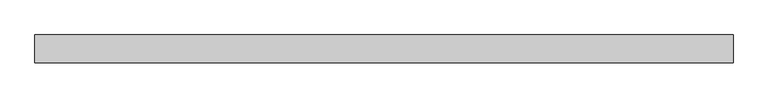
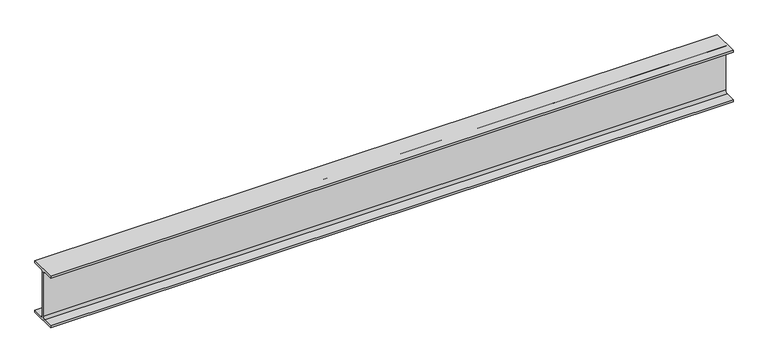
"""IFC4 building model written with IfcOpenShell, lengths in millimetres: beam geometry, 0912_Steel Framing_H-KSD3502 : H_SB_ASB_H-250x125x6x9."""

import ifcopenshell
import ifcopenshell.guid

model = None  # the IFC model being written
_history = None  # IfcOwnerHistory: only IFC2X3 demands one
_inside = {}  # id of a spatial element -> (the spatial element, [elements in it])
_under = {}  # id of a project, library or spatial element -> (it, [spatial elements below it])
_declared = {}  # id of a project -> (the project, [libraries it declares])
_typed = {}  # id of a type object -> (the type object, [elements of that type])
_made_of = {}  # id of a material, layer set ... -> (it, [elements and type objects made of it])


def new_model(schema):
    """Start an empty IFC model of exactly this schema.

    Asked for "IFC4X3", IfcOpenShell would pick the latest addendum, in which some entities
    have other attributes; the version numbers below select the first issue.
    IFC2X3 requires an IfcOwnerHistory on every rooted entity: one is made here for all.
    """
    global model, _history
    if schema == "IFC4X3":
        model = ifcopenshell.file(schema_version=(4, 3, 0, 0))
    else:
        model = ifcopenshell.file(schema=schema)
    _inside.clear()
    _under.clear()
    _declared.clear()
    _typed.clear()
    _made_of.clear()
    _history = None
    if model.schema == "IFC2X3":
        org = make("IfcOrganization", Name="unknown")
        user = make(
            "IfcPersonAndOrganization",
            ThePerson=make("IfcPerson", FamilyName="unknown"),
            TheOrganization=org,
        )
        app = make(
            "IfcApplication",
            ApplicationDeveloper=org,
            Version="unknown",
            ApplicationFullName="unknown",
            ApplicationIdentifier="unknown",
        )
        _history = make(
            "IfcOwnerHistory",
            OwningUser=user,
            OwningApplication=app,
            ChangeAction="ADDED",
            CreationDate=0,
        )
    return model


def make(cls, **values):
    """One entity of the class cls with the attributes given. An attribute that is None is left unset."""
    return model.create_entity(
        cls, **{name: value for name, value in values.items() if value is not None}
    )


def rooted(cls, **values):
    """An entity with a GlobalId (a new one), such as an element, a storey or a relation."""
    return make(cls, GlobalId=ifcopenshell.guid.new(), OwnerHistory=_history, **values)


def si_unit(unit_type, name, prefix=None):
    """IfcSIUnit, for example si_unit("LENGTHUNIT", "METRE", prefix="MILLI")."""
    return make("IfcSIUnit", UnitType=unit_type, Prefix=prefix, Name=name)


def assignment(units):
    """IfcUnitAssignment: the units of a project."""
    return None if units is None else make("IfcUnitAssignment", Units=units)


def point(xyz):
    """IfcCartesianPoint."""
    return None if xyz is None else make("IfcCartesianPoint", Coordinates=xyz)


def direction(xyz):
    """IfcDirection."""
    return None if xyz is None else make("IfcDirection", DirectionRatios=xyz)


def frame(location, z_axis=None, x_axis=None):
    """IfcAxis2Placement3D, a coordinate frame: its origin and axes. An axis left out is left unset."""
    return make(
        "IfcAxis2Placement3D",
        Location=point(location),
        Axis=direction(z_axis),
        RefDirection=direction(x_axis),
    )


def frame_2d(location, x_axis=None):
    """IfcAxis2Placement2D, a coordinate frame in the plane: its origin and x axis."""
    return make(
        "IfcAxis2Placement2D", Location=point(location), RefDirection=direction(x_axis)
    )


def origin():
    """The frame at (0, 0, 0) with its axes left unset."""
    return frame((0.0, 0.0, 0.0))


def place(relative_to, where):
    """IfcLocalPlacement: puts the frame where relative to a parent placement (None: the world)."""
    return make(
        "IfcLocalPlacement", PlacementRelTo=relative_to, RelativePlacement=where
    )


def context(
    kind, dimensions, precision=None, world=None, true_north=None, identifier=None
):
    """IfcGeometricRepresentationContext, for example the 3D "Model" context."""
    return make(
        "IfcGeometricRepresentationContext",
        ContextIdentifier=identifier,
        ContextType=kind,
        CoordinateSpaceDimension=dimensions,
        Precision=precision,
        WorldCoordinateSystem=world,
        TrueNorth=true_north,
    )


def project(units=None, contexts=None):
    """IfcProject with its units and contexts."""
    return rooted(
        "IfcProject",
        Name="project",
        RepresentationContexts=contexts,
        UnitsInContext=assignment(units),
    )


def spatial(cls, under=None, at=None, **own):
    """A site, building, storey or space (cls), placed at a placement, below another one or the project."""
    s = rooted(cls, ObjectPlacement=at, **own)
    if under is not None:
        _under.setdefault(under.id(), (under, []))[1].append(s)
    return s


def polyline(points):
    """IfcPolyline through the points."""
    return make("IfcPolyline", Points=[point(p) for p in points])


def circle_curve(where, radius):
    """IfcCircle in the frame where."""
    return make("IfcCircle", Position=where, Radius=radius)


def trimmed(basis, trim1, trim2, sense, master):
    """IfcTrimmedCurve: the piece of a basis curve between two trims."""
    return make(
        "IfcTrimmedCurve",
        BasisCurve=basis,
        Trim1=trim1,
        Trim2=trim2,
        SenseAgreement=sense,
        MasterRepresentation=master,
    )


def segment(curve, same_sense, transition):
    """IfcCompositeCurveSegment."""
    return make(
        "IfcCompositeCurveSegment",
        Transition=transition,
        SameSense=same_sense,
        ParentCurve=curve,
    )


def composite_curve(segments, self_intersect=None):
    """IfcCompositeCurve: segments joined end to end."""
    return make("IfcCompositeCurve", Segments=segments, SelfIntersect=self_intersect)


def outline(outer, holes=None, kind="AREA"):
    """IfcArbitraryClosedProfileDef: a profile drawn as a closed curve; with holes, ...WithVoids."""
    if holes is None:
        return make("IfcArbitraryClosedProfileDef", ProfileType=kind, OuterCurve=outer)
    return make(
        "IfcArbitraryProfileDefWithVoids",
        ProfileType=kind,
        OuterCurve=outer,
        InnerCurves=holes,
    )


def extrude(swept, where, along, depth):
    """IfcExtrudedAreaSolid: the profile swept, set in the frame where, extruded along a direction by depth."""
    return make(
        "IfcExtrudedAreaSolid",
        SweptArea=swept,
        Position=where,
        ExtrudedDirection=direction(along),
        Depth=depth,
    )


def shape(context_of_items, identifier, shape_type, items):
    """IfcShapeRepresentation: the items that make up one representation, for example the "Body"."""
    return make(
        "IfcShapeRepresentation",
        ContextOfItems=context_of_items,
        RepresentationIdentifier=identifier,
        RepresentationType=shape_type,
        Items=items,
    )


def source(mapping_origin, context_of_items, identifier, shape_type, items):
    """IfcRepresentationMap: a shape defined once, which mapped items show again and again."""
    return make(
        "IfcRepresentationMap",
        MappingOrigin=mapping_origin,
        MappedRepresentation=shape(context_of_items, identifier, shape_type, items),
    )


def transform(
    local_origin,
    x_axis=None,
    y_axis=None,
    z_axis=None,
    scale=None,
    scale2=None,
    scale3=None,
    uniform=True,
):
    """IfcCartesianTransformationOperator3D, or its non-uniform kind. x_axis, y_axis, z_axis: its Axis1, 2, 3."""
    if uniform:
        return make(
            "IfcCartesianTransformationOperator3D",
            Axis1=direction(x_axis),
            Axis2=direction(y_axis),
            LocalOrigin=point(local_origin),
            Scale=scale,
            Axis3=direction(z_axis),
        )
    return make(
        "IfcCartesianTransformationOperator3DnonUniform",
        Axis1=direction(x_axis),
        Axis2=direction(y_axis),
        LocalOrigin=point(local_origin),
        Scale=scale,
        Axis3=direction(z_axis),
        Scale2=scale2,
        Scale3=scale3,
    )


def mapped(mapping_source, mapping_target):
    """IfcMappedItem: shows the shape of a source again, moved by a transform."""
    return make(
        "IfcMappedItem", MappingSource=mapping_source, MappingTarget=mapping_target
    )


def made_of(thing, what):
    """Note that an element or type object is made of a material, layer set ...; save() writes the relation."""
    if what is not None:
        _made_of.setdefault(what.id(), (what, []))[1].append(thing)
    return thing


def element(
    cls,
    number,
    at=None,
    inside=None,
    cuts=None,
    type_object=None,
    material=None,
    context=None,
    identifier="Body",
    shape_type=None,
    held_by="IfcProductDefinitionShape",
    body=None,
    shapes=None,
    **own,
):
    """One element of the class cls, such as IfcWall. Its Tag is "e" and its number.

    at: its placement. inside: the storey or other place that contains it. cuts: it is an
    opening in that element (IfcRelVoidsElement). A single representation is given by context,
    identifier, shape_type and body (its items); several are given by shapes. held_by: the class
    of the entity that holds the representations. save() writes the other relations.
    """
    e = rooted(cls, Tag="e%d" % number, ObjectPlacement=at, **own)
    if body is not None:
        shapes = [shape(context, identifier, shape_type, body)]
    if shapes is not None:
        e.Representation = make(held_by, Representations=shapes)
    if inside is not None:
        _inside.setdefault(inside.id(), (inside, []))[1].append(e)
    if cuts is not None:
        rooted(
            "IfcRelVoidsElement", RelatingBuildingElement=cuts, RelatedOpeningElement=e
        )
    if type_object is not None:
        _typed.setdefault(type_object.id(), (type_object, []))[1].append(e)
    return made_of(e, material)


def aggregate(whole, parts):
    """IfcRelAggregates: a whole, such as a stair, and the parts it consists of."""
    return rooted("IfcRelAggregates", RelatingObject=whole, RelatedObjects=parts)


def save(model, path):
    """Write the relations noted so far, then the file.

    IfcRelAggregates (storeys below a building ...), IfcRelContainedInSpatialStructure (elements
    in a storey), IfcRelDefinesByType, IfcRelAssociatesMaterial and IfcRelDeclares: one each for
    every whole, place, type object, material and project.
    """
    for whole, parts in _under.values():
        aggregate(whole, parts)
    for where, things in _inside.values():
        rooted(
            "IfcRelContainedInSpatialStructure",
            RelatedElements=things,
            RelatingStructure=where,
        )
    for kind, things in _typed.values():
        rooted("IfcRelDefinesByType", RelatedObjects=things, RelatingType=kind)
    for what, things in _made_of.values():
        rooted("IfcRelAssociatesMaterial", RelatedObjects=things, RelatingMaterial=what)
    for by, libraries in _declared.values():
        rooted("IfcRelDeclares", RelatingContext=by, RelatedDefinitions=libraries)
    model.write(path)


def beam_d1df00b5(model_context):
    return source(origin(), model_context, "Body", "SweptSolid", [
        extrude(outline(composite_curve([segment(polyline([(62.5, -116.0), (62.5, -125.0), (-62.5, -125.0), (-62.5, -116.0), (-15.0, -116.0)]), True, "CONTINUOUS"), segment(trimmed(circle_curve(frame_2d((-15.0, -104.0)), 12.0), [point((-15.0, -116.0))], [point((-3.0, -104.0))], True, "CARTESIAN"), True, "CONTINUOUS"), segment(polyline([(-3.0, -104.0), (-3.0, 104.0)]), True, "CONTINUOUS"), segment(trimmed(circle_curve(frame_2d((-15.0, 104.0)), 12.0), [point((-3.0, 104.0))], [point((-15.0, 116.0))], True, "CARTESIAN"), True, "CONTINUOUS"), segment(polyline([(-15.0, 116.0), (-62.5, 116.0), (-62.5, 125.0), (62.5, 125.0), (62.5, 116.0), (15.0, 116.0)]), True, "CONTINUOUS"), segment(trimmed(circle_curve(frame_2d((15.0, 104.0)), 12.0), [point((15.0, 116.0))], [point((3.0, 104.0))], True, "CARTESIAN"), True, "CONTINUOUS"), segment(polyline([(3.0, 104.0), (3.0, -104.0)]), True, "CONTINUOUS"), segment(trimmed(circle_curve(frame_2d((15.0, -104.0)), 12.0), [point((3.0, -104.0))], [point((15.0, -116.0))], True, "CARTESIAN"), True, "CONTINUOUS"), segment(polyline([(15.0, -116.0), (62.5, -116.0)]), True, "CONTINUOUS")], self_intersect=False)), frame((-1654.8, 0.0, 0.0), z_axis=(1.0, 0.0, 0.0), x_axis=(0.0, 1.0, 0.0)), (0.0, 0.0, 1.0), 3149.3360727),
    ])


if __name__ == "__main__":
    model = new_model("IFC4")
    model_context = context("Model", 3, world=origin())
    ifc_project = project(units=[si_unit("LENGTHUNIT", "METRE", prefix="MILLI")], contexts=[model_context])
    site = spatial("IfcSite", under=ifc_project)
    building = spatial("IfcBuilding", under=site)
    placement = place(None, origin())
    beam_shape = beam_d1df00b5(model_context)
    element("IfcBeam", 1, ObjectType="0912_Steel Framing_H-KSD3502 : H_SB_ASB_H-250x125x6x9", at=placement, inside=building, context=model_context, shape_type="MappedRepresentation", body=[
        mapped(beam_shape, transform((0.0, 0.0, 0.0), x_axis=(1.0, 0.0, 0.0), y_axis=(0.0, 1.0, 0.0), z_axis=(0.0, 0.0, 1.0))),
    ])
    save(model, "model.ifc")

# Revit data of these elements
# Type "0912_Steel Framing_H-KSD3502 : H_SB_ASB_H-250x125x6x9"
#   H_WM Code_1 = "S01AA003-00001 | Main Steel Structure Fabrication Work | Shelter/Building | Light Steel - Standard (30KG/M>Weight) | Material: (   )"
#   H_WM Code_2 = "S03AA029-00001 | Main Steel Structure Erection Work | Shelter/Building | Light Steel (30KG/M>Weight) | Material: (   )"
#   H_WM Code_3 = "S01AA010-00001 | Main Steel Structure Fabrication Work | Shelter/Building | Steel Painting/Coating | for Non-Fireproofed Steel Surface, Surface Preparation, Primer, Second & Final Coat | Material: (   )"
#   H_Q'ty Cal Type Tag = "SB-Q2"
#   Width = 12.5 cm
#   Web Thickness = 0.6 cm
#   Web Fillet = 1.2 cm
#   Warping Constant = 42539.8 cm⁶
#   W = 0
#   Torsional Moment of Inertia = 7.8102 cm⁴
#   Section Area = 37.66 cm²
#   Plastic Modulus weak axis = 73.1 cm³
#   Plastic Modulus strong axis = 366.0 cm³
#   Perimeter = 0.97 m²/m
#   Nominal Weight = 29.60 kgf/m
#   Moment of Inertia weak axis = 294.00 cm⁴
#   Moment of Inertia strong axis = 4050.00 cm⁴
#   Height = 25.0 cm
#   Flange Thickness = 0.9 cm
#   Elastic Modulus weak axis = 47.0 cm³
#   Elastic Modulus strong axis = 324.0 cm³
#   Centroid Vertical = 12.5 cm
#   Centroid Horizontal = 6.25 cm
#   Ix = 40500000
#   Length [instance default] = 1.5240 m
#   Zx = 366000
#   b = 0.1250 m
#   h = 0.2500 m
#   r = 0.0120 m
#   s = 0.0060 m
#   t = 0.0090 m
#   A = 0.003766 m²
#   Structural Material [instance default] = Steel, 45-345
#   Assembly Code = ""
# Element 1 (IfcBeam, "0912_Steel Framing_H-KSD3502 : H_SB_ASB_H-250x125x6x9")
#   Structural Material = none
# Materials
#   "Steel, 45-345": class "Metal", colour RGB 189 187 185, transparency 0, Description = "Steel 345 MPa", Cost = 0
